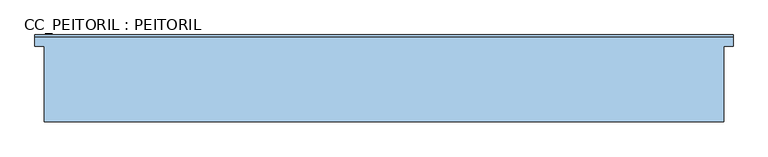
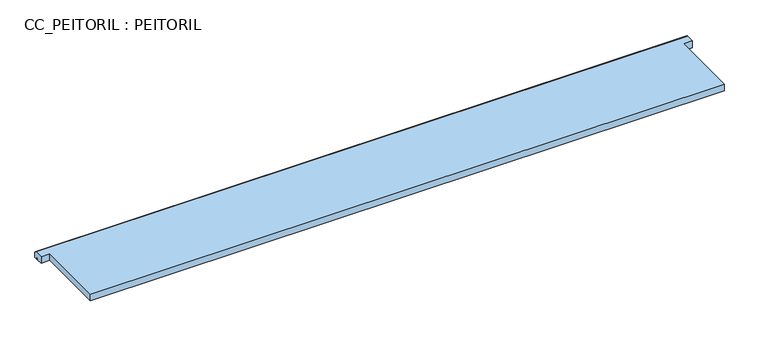
"""IFC4 building model written with IfcOpenShell, lengths in millimetres: window geometry, CC_PEITORIL : PEITORIL."""

from ifc_helpers import new_model, si_unit, frame, origin, place, context, project, spatial, circle_curve, source, transform, mapped, element, save
from ifc_brep_helpers import plane_surface, cylinder_surface, advanced_brep


def cc_peitoril_peitoril_f71d5caf(model_context):
    return source(origin(), model_context, "Body", "AdvancedBrep", [
        advanced_brep(
        [(-900.0, 100.0, 1500.0), (-900.0, -100.0, 1500.0), (900.0, -100.0, 1500.0), (900.0, 100.0, 1500.0), (925.0, 100.0, 1500.0), (925.0, 123.4916648, 1500.0), (-925.0, 123.4916648, 1500.0), (-925.0, 100.0, 1500.0), (-900.0, 100.0, 1480.0), (-925.0, 100.0, 1480.0), (-925.0, 115.0, 1480.0), (925.0, 115.0, 1480.0), (925.0, 100.0, 1480.0), (900.0, 100.0, 1480.0), (900.0, -100.0, 1480.0), (-900.0, -100.0, 1480.0), (-925.0, 130.0, 1480.0), (925.0, 130.0, 1480.0), (925.0, 120.0, 1480.0), (-925.0, 120.0, 1480.0), (925.0, 115.0, 1485.0), (925.0, 120.0, 1485.0), (925.0, 130.0, 1493.4916648), (-925.0, 130.0, 1493.4916648), (-925.0, 120.0, 1485.0), (-925.0, 115.0, 1485.0)],
        [
            (0, 1),
            (1, 2),
            (2, 3),
            (3, 4),
            (4, 5),
            (5, 6),
            (6, 7),
            (7, 0),
            (8, 9),
            (9, 10),
            (10, 11),
            (11, 12),
            (12, 13),
            (13, 14),
            (14, 15),
            (15, 8),
            (16, 17),
            (17, 18),
            (18, 19),
            (19, 16),
            (0, 8),
            (15, 1),
            (14, 2),
            (13, 3),
            (12, 4),
            (11, 20),
            (20, 21),
            (21, 18),
            (17, 22),
            (22, 5, circle_curve(frame((925.0, 123.4916648, 1493.4916648), z_axis=(1.0, 0.0, 0.0), x_axis=(0.0, -1.0, 0.0)), 6.5083352)),
            (16, 23),
            (23, 22),
            (9, 7),
            (6, 23, circle_curve(frame((-925.0, 123.4916648, 1493.4916648), z_axis=(-1.0, 0.0, 0.0), x_axis=(0.0, -1.0, 0.0)), 6.5083352)),
            (19, 24),
            (24, 25),
            (25, 10),
            (24, 21),
            (20, 25),
        ],
        [
            plane_surface(frame((-900.0, -100.0, 1500.0), z_axis=(0.0, 0.0, 1.0), x_axis=(0.0, -1.0, 0.0))),
            plane_surface(frame((-900.0, -100.0, 1480.0), z_axis=(0.0, 0.0, -1.0), x_axis=(0.0, 1.0, 0.0))),
            plane_surface(frame((-900.0, 100.0, 1500.0), z_axis=(-1.0, 0.0, 0.0), x_axis=(0.0, 0.0, -1.0))),
            plane_surface(frame((-900.0, -100.0, 1500.0), z_axis=(0.0, -1.0, 0.0), x_axis=(0.0, 0.0, -1.0))),
            plane_surface(frame((900.0, -100.0, 1500.0), z_axis=(1.0, 0.0, 0.0), x_axis=(0.0, 0.0, -1.0))),
            plane_surface(frame((900.0, 100.0, 1500.0), z_axis=(0.0, -1.0, 0.0), x_axis=(0.0, 0.0, -1.0))),
            plane_surface(frame((925.0, 100.0, 1500.0), z_axis=(1.0, 0.0, 0.0), x_axis=(0.0, 0.0, -1.0))),
            plane_surface(frame((925.0, 130.0, 1500.0), z_axis=(0.0, 1.0, 0.0), x_axis=(0.0, 0.0, -1.0))),
            plane_surface(frame((-925.0, 130.0, 1500.0), z_axis=(-1.0, 0.0, 0.0), x_axis=(0.0, 0.0, -1.0))),
            plane_surface(frame((-925.0, 100.0, 1500.0), z_axis=(0.0, -1.0, 0.0), x_axis=(0.0, 0.0, -1.0))),
            cylinder_surface(frame((925.0, 123.4916648, 1493.4916648), z_axis=(-1.0, 0.0, 0.0), x_axis=(0.0, -1.0, 0.0)), 6.5083352),
            plane_surface(frame((-925.0, 115.0, 1485.0), z_axis=(0.0, 0.0, -1.0), x_axis=(1.0, 0.0, 0.0))),
            plane_surface(frame((-925.0, 120.0, 1485.0), z_axis=(0.0, -1.0, 0.0), x_axis=(1.0, 0.0, 0.0))),
            plane_surface(frame((-925.0, 115.0, 1480.0), z_axis=(0.0, 1.0, 0.0), x_axis=(1.0, 0.0, 0.0))),
        ],
        [
            (0, [[1, 2, 3, 4, 5, 6, 7, 8]]),
            (1, [[9, 10, 11, 12, 13, 14, 15, 16]]),
            (1, [[17, 18, 19, 20]]),
            (2, [[-1, 21, -16, 22]]),
            (3, [[-2, -22, -15, 23]]),
            (4, [[-3, -23, -14, 24]]),
            (5, [[-4, -24, -13, 25]]),
            (6, [[-25, -12, 26, 27, 28, -18, 29, 30, -5]]),
            (7, [[-17, 31, 32, -29]]),
            (8, [[33, -7, 34, -31, -20, 35, 36, 37, -10]]),
            (9, [[-8, -33, -9, -21]]),
            (10, [[-6, -30, -32, -34]]),
            (11, [[38, -27, 39, -36]]),
            (12, [[-38, -35, -19, -28]]),
            (13, [[-39, -26, -11, -37]]),
        ],
    ),
    ])


if __name__ == "__main__":
    model = new_model("IFC4")
    model_context = context("Model", 3, world=origin())
    ifc_project = project(units=[si_unit("LENGTHUNIT", "METRE", prefix="MILLI")], contexts=[model_context])
    site = spatial("IfcSite", under=ifc_project)
    building = spatial("IfcBuilding", under=site)
    placement = place(None, origin())
    cc_peitoril_peitoril_shape = cc_peitoril_peitoril_f71d5caf(model_context)
    element("IfcWindow", 1, ObjectType="CC_PEITORIL : PEITORIL", at=placement, inside=building, context=model_context, shape_type="MappedRepresentation", body=[
        mapped(cc_peitoril_peitoril_shape, transform((0.0, 0.0, 0.0), x_axis=(1.0, 0.0, 0.0), y_axis=(0.0, 1.0, 0.0), z_axis=(0.0, 0.0, 1.0))),
    ])
    save(model, "model.ifc")

# Revit data of these elements
# Type "CC_PEITORIL : PEITORIL"
#   Type Mark = "PEITORIL"
#   Analytic Construction = "<Nenhum>"
#   Largura da pedra [instance default] = 0.26 m
#   Interna [instance default] = 0.08 m
#   Externa [instance default] = 0.008142 m
#   Extensão Exterior [instance default] = 0.03 m
#   Extensão Exterior Esquerda [instance default] = 0.085058 m
#   Extensão Exterior Direita [instance default] = 0.10 m
#   Espessura [instance default] = 0.02 m
#   Comprimento [instance default] = 1.00 m
#   Altura-padrão do peitoril = 1.48 m
#   ----EXTENSÃO---- [instance default] = 0.00 m
#   ----DEMAIS---- [instance default] = 0.00 m
#   Peitoril [instance default] = none
#   Rough Width = 0
#   Rough Height = 0
#   Height = 0
#   Wall Closure = (empty or 0)
#   Width = 0
# Element 1 (IfcWindow, "CC_PEITORIL : PEITORIL")
#   Interna = 0.00 m
#   Externa = 0.00 m
#   Extensão Exterior Esquerda = 0.025 m
#   Extensão Exterior Direita = 0.025 m
#   Comprimento = 1.80 m
#   Peitoril = .GRANITO BRANCO ITAÚNAS
#   Materials on its faces: ".GRANITO BRANCO ITAÚNAS"
# Materials
#   ".GRANITO BRANCO ITAÚNAS": class ".CC_PEDRA REVEST.", colour RGB 202 195 174, transparency 0, Description = "Granito branco Itaúnas", Uso = "Pedra", Cost = 0
